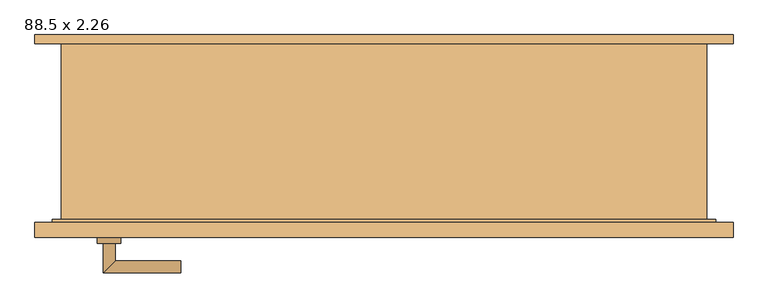
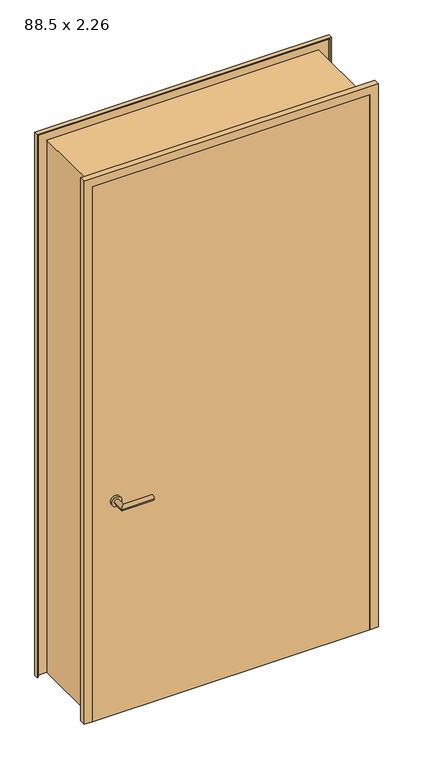
"""IFC4 building model written with IfcOpenShell, lengths in millimetres: door geometry, Drehflügel 1-flg - Stahlzarge : 88.5 x 2.26."""

from ifc_helpers import new_model, si_unit, point, frame, frame_2d, origin, place, context, project, spatial, polyline, circle_curve, ellipse_curve, trimmed, segment, composite_curve, outline, extrude, faceted_brep, source, transform, mapped, element, save
from ifc_brep_helpers import plane_surface, cylinder_surface, advanced_brep


def door_88_5_x_2_26_5622a663(model_context):
    return source(origin(), model_context, "Body", "SolidModel", [
        advanced_brep(
        [(-471.4, -139.4346141, 1000.0), (-451.4, -139.4346141, 1000.0), (-451.4, -89.4346141, 1000.0), (-471.4, -69.4346141, 1000.0), (-341.4, -69.4346141, 1000.0), (-341.4, -89.4346141, 1000.0)],
        [
            (0, 1, circle_curve(frame((-461.4, -139.4346141, 1000.0), z_axis=(0.0, -1.0, 0.0), x_axis=(1.0, 0.0, 0.0)), 10.0)),
            (1, 0, circle_curve(frame((-461.4, -139.4346141, 1000.0), z_axis=(0.0, -1.0, 0.0), x_axis=(1.0, 0.0, 0.0)), 10.0)),
            (1, 2),
            (2, 3, ellipse_curve(frame((-461.4, -79.4346141, 1000.0), z_axis=(-0.7071067811865385, -0.7071067811865565, 0.0), x_axis=(0.7071067811865563, -0.7071067811865386, 0.0)), 14.1421356, 10.0)),
            (3, 0),
            (3, 2, ellipse_curve(frame((-461.4, -79.4346141, 1000.0), z_axis=(-0.7071067811865385, -0.7071067811865565, 0.0), x_axis=(0.7071067811865563, -0.7071067811865386, 0.0)), 14.1421356, 10.0)),
            (4, 5, circle_curve(frame((-341.4, -79.4346141, 1000.0), z_axis=(1.0, 0.0, 0.0), x_axis=(0.0, -1.0, 0.0)), 10.0)),
            (5, 4, circle_curve(frame((-341.4, -79.4346141, 1000.0), z_axis=(1.0, 0.0, 0.0), x_axis=(0.0, -1.0, 0.0)), 10.0)),
            (2, 5),
            (4, 3),
        ],
        [
            plane_surface(frame((-461.4, -139.4346141, -287.7526403), z_axis=(0.0, -1.0, 0.0), x_axis=(0.0, 0.0, 1.0))),
            cylinder_surface(frame((-461.4, -139.4346141, 1000.0), z_axis=(0.0, -1.0, 0.0), x_axis=(1.0, 0.0, 0.0)), 10.0),
            plane_surface(frame((-341.4, -79.4346141, -287.7526403), z_axis=(1.0, 0.0, 0.0), x_axis=(0.0, 0.0, 1.0))),
            cylinder_surface(frame((-461.4, -79.4346141, 1000.0), z_axis=(-1.0, 0.0, 0.0), x_axis=(0.0, -1.0, 0.0)), 10.0),
        ],
        [
            (0, [[1, 2]]),
            (1, [[3, 4, 5, -2]]),
            (1, [[-5, 6, -3, -1]]),
            (2, [[7, 8]]),
            (3, [[9, -7, 10, -4]]),
            (3, [[-10, -8, -9, -6]]),
        ],
    ),
        advanced_brep(
        [(-451.4, -199.4346141, 1000.0), (-471.4, -199.4346141, 1000.0), (-471.4, -249.4346141, 1000.0), (-451.4, -229.4346141, 1000.0), (-341.4, -229.4346141, 1000.0), (-341.4, -249.4346141, 1000.0)],
        [
            (0, 1, circle_curve(frame((-461.4, -199.4346141, 1000.0), z_axis=(0.0, 1.0, 0.0), x_axis=(-1.0, 0.0, 0.0)), 10.0)),
            (1, 0, circle_curve(frame((-461.4, -199.4346141, 1000.0), z_axis=(0.0, 1.0, 0.0), x_axis=(-1.0, 0.0, 0.0)), 10.0)),
            (1, 2),
            (2, 3, ellipse_curve(frame((-461.4, -239.4346141, 1000.0), z_axis=(-0.7071067811865475, 0.7071067811865475, 0.0), x_axis=(0.7071067811865474, 0.7071067811865476, 0.0)), 14.1421356, 10.0)),
            (3, 0),
            (3, 2, ellipse_curve(frame((-461.4, -239.4346141, 1000.0), z_axis=(-0.7071067811865475, 0.7071067811865475, 0.0), x_axis=(0.7071067811865474, 0.7071067811865476, 0.0)), 14.1421356, 10.0)),
            (4, 5, circle_curve(frame((-341.4, -239.4346141, 1000.0), z_axis=(1.0, 0.0, 0.0), x_axis=(0.0, -1.0, 0.0)), 10.0)),
            (5, 4, circle_curve(frame((-341.4, -239.4346141, 1000.0), z_axis=(1.0, 0.0, 0.0), x_axis=(0.0, -1.0, 0.0)), 10.0)),
            (2, 5),
            (4, 3),
        ],
        [
            plane_surface(frame((-461.4, -199.4346141, -287.7526403), z_axis=(0.0, 1.0, 0.0), x_axis=(0.0, 0.0, 1.0))),
            cylinder_surface(frame((-461.4, -199.4346141, 1000.0), z_axis=(0.0, 1.0, 0.0), x_axis=(-1.0, 0.0, 0.0)), 10.0),
            plane_surface(frame((-341.4, -239.4346141, -287.7526403), z_axis=(1.0, 0.0, 0.0), x_axis=(0.0, 0.0, 1.0))),
            cylinder_surface(frame((-461.4, -239.4346141, 1000.0), z_axis=(-1.0, 0.0, 0.0), x_axis=(0.0, -1.0, 0.0)), 10.0),
        ],
        [
            (0, [[1, 2]]),
            (1, [[3, 4, 5, -2]]),
            (1, [[-5, 6, -3, -1]]),
            (2, [[7, 8]]),
            (3, [[9, -7, 10, -4]]),
            (3, [[-10, -8, -9, -6]]),
        ],
    ),
        extrude(outline(composite_curve([segment(trimmed(circle_curve(frame_2d((1000.0, -461.4)), 20.0), [point((1000.0, -481.4))], [point((1000.0, -441.4))], False, "CARTESIAN"), True, "CONTINUOUS"), segment(trimmed(circle_curve(frame_2d((1000.0, -461.4)), 20.0), [point((1000.0, -441.4))], [point((1000.0, -481.4))], False, "CARTESIAN"), True, "CONTINUOUS")], self_intersect=False)), frame((0.0, -139.4346141, 0.0), z_axis=(0.0, 1.0, 0.0), x_axis=(0.0, 0.0, 1.0)), (0.0, 0.0, 1.0), 10.0),
        extrude(outline(composite_curve([segment(trimmed(circle_curve(frame_2d((1000.0, -461.4)), 20.0), [point((1000.0, -481.4))], [point((1000.0, -441.4))], False, "CARTESIAN"), True, "CONTINUOUS"), segment(trimmed(circle_curve(frame_2d((1000.0, -461.4)), 20.0), [point((1000.0, -441.4))], [point((1000.0, -481.4))], False, "CARTESIAN"), True, "CONTINUOUS")], self_intersect=False)), frame((0.0, -199.4346141, 0.0), z_axis=(0.0, 1.0, 0.0), x_axis=(0.0, 0.0, 1.0)), (0.0, 0.0, 1.0), 10.0),
        extrude(outline(polyline([(551.4, -164.4346141), (551.4, -189.4346141), (-551.4, -189.4346141), (-551.4, -164.4346141), (551.4, -164.4346141)])), frame((0.0, 0.0, 100.0), z_axis=(0.0, 0.0, 1.0), x_axis=(1.0, 0.0, 0.0)), (0.0, 0.0, 1.0), 2250.0),
        faceted_brep([(585.8603207, 150.5653859, 100.0), (585.8603207, 135.5653859, 100.0), (580.8603207, 135.5653859, 100.0), (580.8603207, 145.5653859, 100.0), (541.4, 145.5653859, 100.0), (541.4, -159.4346141, 100.0), (556.4, -159.4346141, 100.0), (556.4, -184.4346141, 100.0), (580.8603207, -184.4346141, 100.0), (580.8603207, -164.4346141, 100.0), (585.8603207, -164.4346141, 100.0), (585.8603207, -189.4346141, 100.0), (551.4, -189.4346141, 100.0), (551.4, -164.4346141, 100.0), (536.4, -164.4346141, 100.0), (536.4, 150.5653859, 100.0), (536.4, 150.5653859, 2335.0), (-536.4, 150.5653859, 2335.0), (-536.4, 150.5653859, 100.0), (-585.8603207, 150.5653859, 100.0), (-585.8603207, 150.5653859, 2384.4603207), (585.8603207, 150.5653859, 2384.4603207), (536.4, -164.4346141, 2335.0), (551.4, -164.4346141, 2350.0), (-551.4, -164.4346141, 2350.0), (-551.4, -164.4346141, 100.0), (-536.4, -164.4346141, 100.0), (-536.4, -164.4346141, 2335.0), (551.4, -189.4346141, 2350.0), (585.8603207, -189.4346141, 2384.4603207), (-585.8603207, -189.4346141, 2384.4603207), (-585.8603207, -189.4346141, 100.0), (-551.4, -189.4346141, 100.0), (-551.4, -189.4346141, 2350.0), (585.8603207, -164.4346141, 2384.4603207), (580.8603207, -164.4346141, 2379.4603207), (-580.8603207, -164.4346141, 2379.4603207), (-580.8603207, -164.4346141, 100.0), (-585.8603207, -164.4346141, 100.0), (-585.8603207, -164.4346141, 2384.4603207), (580.8603207, -184.4346141, 2379.4603207), (556.4, -184.4346141, 2355.0), (-556.4, -184.4346141, 2355.0), (-556.4, -184.4346141, 100.0), (-580.8603207, -184.4346141, 100.0), (-580.8603207, -184.4346141, 2379.4603207), (556.4, -159.4346141, 2355.0), (541.4, -159.4346141, 2340.0), (-541.4, -159.4346141, 2340.0), (-541.4, -159.4346141, 100.0), (-556.4, -159.4346141, 100.0), (-556.4, -159.4346141, 2355.0), (541.4, 145.5653859, 2340.0), (580.8603207, 145.5653859, 2379.4603207), (-580.8603207, 145.5653859, 2379.4603207), (-580.8603207, 145.5653859, 100.0), (-541.4, 145.5653859, 100.0), (-541.4, 145.5653859, 2340.0), (580.8603207, 135.5653859, 2379.4603207), (585.8603207, 135.5653859, 2384.4603207), (-585.8603207, 135.5653859, 2384.4603207), (-585.8603207, 135.5653859, 100.0), (-580.8603207, 135.5653859, 100.0), (-580.8603207, 135.5653859, 2379.4603207)], [[[0, 1, 2, 3, 4, 5, 6, 7, 8, 9, 10, 11, 12, 13, 14, 15]], [[15, 16, 17, 18, 19, 20, 21, 0]], [[14, 22, 16, 15]], [[13, 23, 24, 25, 26, 27, 22, 14]], [[12, 28, 23, 13]], [[11, 29, 30, 31, 32, 33, 28, 12]], [[10, 34, 29, 11]], [[9, 35, 36, 37, 38, 39, 34, 10]], [[8, 40, 35, 9]], [[7, 41, 42, 43, 44, 45, 40, 8]], [[6, 46, 41, 7]], [[5, 47, 48, 49, 50, 51, 46, 6]], [[4, 52, 47, 5]], [[3, 53, 54, 55, 56, 57, 52, 4]], [[2, 58, 53, 3]], [[1, 59, 60, 61, 62, 63, 58, 2]], [[0, 21, 59, 1]], [[20, 19, 61, 60]], [[19, 18, 26, 25, 32, 31, 38, 37, 44, 43, 50, 49, 56, 55, 62, 61]], [[27, 26, 18, 17]], [[33, 32, 25, 24]], [[39, 38, 31, 30]], [[45, 44, 37, 36]], [[51, 50, 43, 42]], [[57, 56, 49, 48]], [[63, 62, 55, 54]], [[22, 27, 17, 16]], [[28, 33, 24, 23]], [[34, 39, 30, 29]], [[40, 45, 36, 35]], [[46, 51, 42, 41]], [[52, 57, 48, 47]], [[58, 63, 54, 53]], [[21, 20, 60, 59]]]),
    ])


if __name__ == "__main__":
    model = new_model("IFC4")
    model_context = context("Model", 3, world=origin())
    ifc_project = project(units=[si_unit("LENGTHUNIT", "METRE", prefix="MILLI")], contexts=[model_context])
    site = spatial("IfcSite", under=ifc_project)
    building = spatial("IfcBuilding", under=site)
    placement = place(None, origin())
    door_88_5_x_2_26_shape = door_88_5_x_2_26_5622a663(model_context)
    element("IfcDoor", 1, ObjectType="Drehflügel 1-flg - Stahlzarge : 88.5 x 2.26", at=placement, inside=building, context=model_context, shape_type="MappedRepresentation", body=[
        mapped(door_88_5_x_2_26_shape, transform((0.0, 0.0, 0.0), x_axis=(1.0, 0.0, 0.0), y_axis=(0.0, 1.0, 0.0), z_axis=(0.0, 0.0, 1.0))),
    ])
    save(model, "model.ifc")

# Revit data of these elements
# Type "Drehflügel 1-flg - Stahlzarge : 88.5 x 2.26"
#   Construction Type Id = "MDOOR"
#   Type Mark = "20"
#   Operation = "SingleSwingRight"
#   Keynote = "16.03"
#   Analytic Construction = "Metall"
#   Thermal Resistance (R) = 0.270117 (m²·K)/W
#   Heat Transfer Coefficient (U) = 3.7021 W/(m²·K)
#   Rough Width = 1.1228 m
#   Rough Height [instance default] = 2.360 m
#   Höhe Türgriff [instance default] = 0.900 m
#   Height = 2.260 m
#   Fußbodenaufbau [instance default] = 0.100 m
#   Width = 1.1228 m
#   Sichtbarkeit Sturzlinien [instance default] = yes
#   Türgriff auswählen [instance default] = element 221079
#   Türgriff [instance default] = none
#   Türflügel [instance default] = none
#   Rahmen/Pfosten [instance default] = Metall - Lackiert - Grau
#   Visual Light Transmittance = 0
#   Solar Heat Gain Coefficient = 0
#   Function = (empty or 0)
#   Wall Closure = (empty or 0)
# Element 1 (IfcDoor, "Drehflügel 1-flg - Stahlzarge : 88.5 x 2.26")
#   Materials on its faces: "Metall - Lackiert - Grau", "Metall - Chrom", "Holz - Birke"
# Materials
#   "Metall - Lackiert - Grau": class "Farbe 1", colour RGB 98 98 98, transparency 0, Cost = 0
#   "Metall - Chrom": class "Metall", colour RGB 247 247 247, transparency 0, Cost = 0
#   "Holz - Birke": class "Holz", colour RGB 213 164 103, transparency 0, Cost = 0
